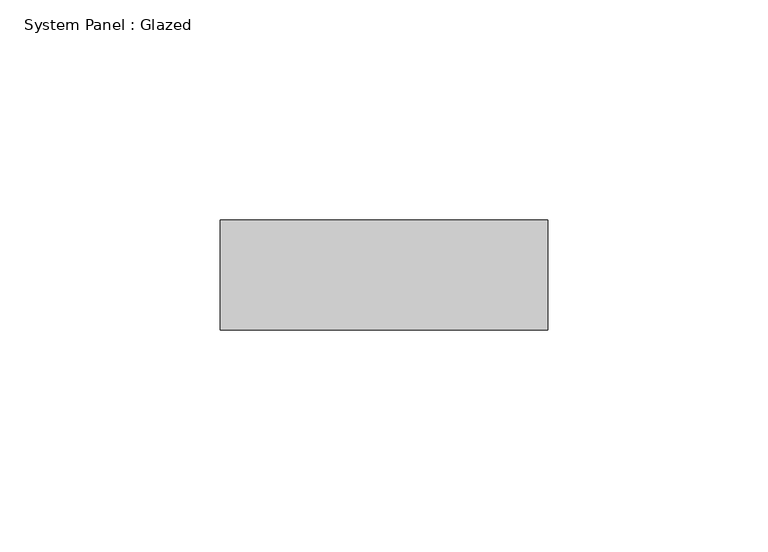
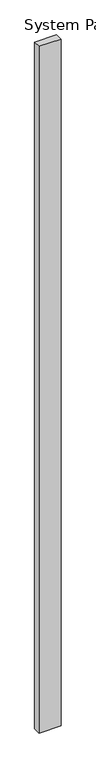
"""IFC4 building model written with IfcOpenShell, lengths in millimetres: plate geometry, System Panel : Glazed."""

from ifc_helpers import new_model, si_unit, origin, origin_with_axes, place, context, project, spatial, polyline, outline, extrude, source, transform, mapped, element, save


def system_panel_glazed_54eb7814(model_context):
    return source(origin(), model_context, "Body", "SweptSolid", [
        extrude(outline(polyline([(37.2092572, 24.5), (-37.2092572, 24.5), (-37.2092572, 49.5), (37.2092572, 49.5), (37.2092572, 24.5)])), origin_with_axes(), (0.0, 0.0, 1.0), 2450.0),
    ])


if __name__ == "__main__":
    model = new_model("IFC4")
    model_context = context("Model", 3, world=origin())
    ifc_project = project(units=[si_unit("LENGTHUNIT", "METRE", prefix="MILLI")], contexts=[model_context])
    site = spatial("IfcSite", under=ifc_project)
    building = spatial("IfcBuilding", under=site)
    placement = place(None, origin())
    system_panel_glazed_shape = system_panel_glazed_54eb7814(model_context)
    element("IfcPlate", 1, ObjectType="System Panel : Glazed", at=placement, inside=building, context=model_context, shape_type="MappedRepresentation", body=[
        mapped(system_panel_glazed_shape, transform((0.0, 0.0, 0.0), x_axis=(1.0, 0.0, 0.0), y_axis=(0.0, 1.0, 0.0), z_axis=(0.0, 0.0, 1.0))),
    ])
    save(model, "model.ifc")

# Revit data of these elements
# Type "System Panel : Glazed"
#   Keynote = "H11"
#   Construction Type Id = "GSP4R"
#   Analytic Construction = "1/8 in Pilkington single glazing"
#   Visual Light Transmittance = 0.9
#   Solar Heat Gain Coefficient = 0.86
#   Heat Transfer Coefficient (U) = 6.7069 W/(m²·K)
# Element 1 (IfcPlate, "System Panel : Glazed")
#   Materials on its faces: "Glass"
# Materials
#   "Glass": class "Glass", colour RGB 0 128 192, transparency 0.9, Description = "Soda Lime Glass", Cost = 0
